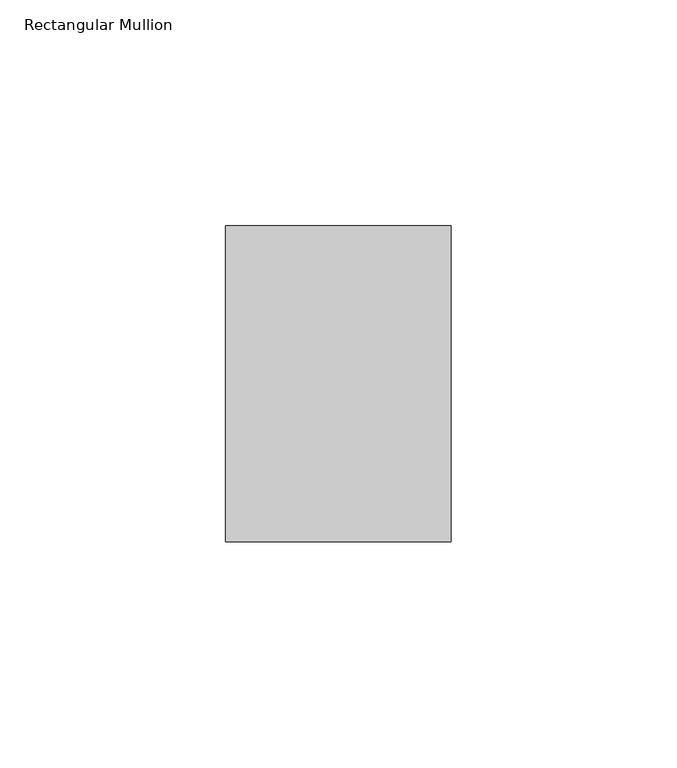
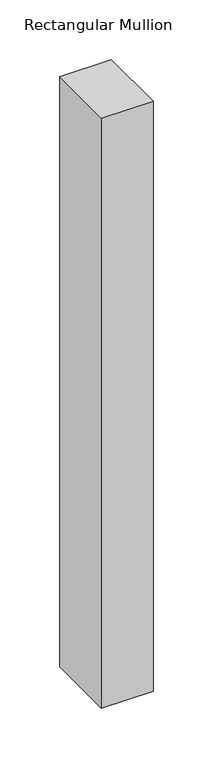
"""IFC4 building model written with IfcOpenShell, lengths in millimetres: member geometry, Rectangular Mullion : WWm-25x70-35mmOffset."""

from ifc_helpers import new_model, si_unit, frame, origin, place, context, project, spatial, polyline, outline, extrude, source, transform, mapped, element, save


def rectangular_mullion_4ac823b4(model_context):
    return source(origin(), model_context, "Body", "SweptSolid", [
        extrude(outline(polyline([(0.0, 0.0), (0.0, -70.0), (-50.0, -70.0), (-50.0, 0.0), (0.0, 0.0)])), frame((0.0, 0.0, -604.0), z_axis=(0.0, 0.0, 1.0), x_axis=(1.0, 0.0, 0.0)), (0.0, 0.0, 1.0), 604.0),
    ])


if __name__ == "__main__":
    model = new_model("IFC4")
    model_context = context("Model", 3, world=origin())
    ifc_project = project(units=[si_unit("LENGTHUNIT", "METRE", prefix="MILLI")], contexts=[model_context])
    site = spatial("IfcSite", under=ifc_project)
    building = spatial("IfcBuilding", under=site)
    placement = place(None, origin())
    rectangular_mullion_shape = rectangular_mullion_4ac823b4(model_context)
    element("IfcMember", 1, ObjectType="Rectangular Mullion : WWm-25x70-35mmOffset", at=placement, inside=building, context=model_context, shape_type="MappedRepresentation", body=[
        mapped(rectangular_mullion_shape, transform((0.0, 0.0, 0.0), x_axis=(1.0, 0.0, 0.0), y_axis=(0.0, 1.0, 0.0), z_axis=(0.0, 0.0, 1.0))),
    ])
    save(model, "model.ifc")

# Revit data of these elements
# Type "Rectangular Mullion : WWm-25x70-35mmOffset"
#   built-in parameter 1007351 = 0.114829 (stored number, unit not read)
#   built-in parameter 1007304 = 0.229659 (stored number, unit not read)
#   built-in parameter 1007301 = 0.082021 (stored number, unit not read)
#   built-in parameter 1007300 = 0.082021 (stored number, unit not read)
# Element 1 (IfcMember, "Rectangular Mullion : WWm-25x70-35mmOffset")
#   Materials on its faces: "WW-EC-RGB-Mullion"
# Materials
#   "WW-EC-RGB-Mullion": class "Generic", colour RGB 255 255 255, transparency 0, Comments = "If region requests black mullions, switch asset color to RGB 25-25-25", Description = "Generic Color", Cost = 0
